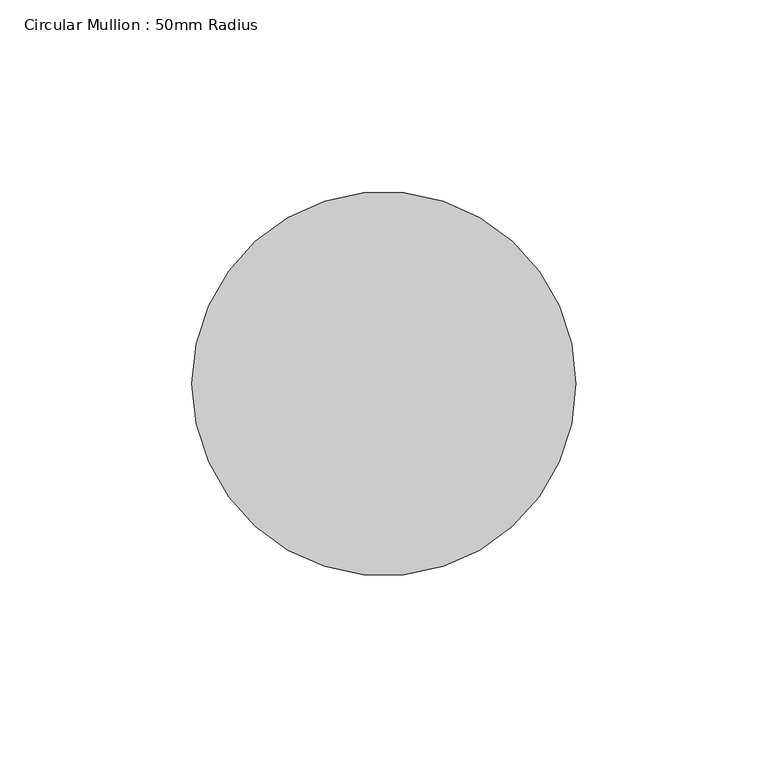
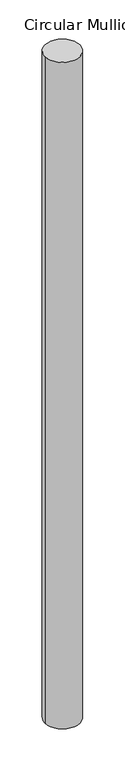
"""IFC4 building model written with IfcOpenShell, lengths in millimetres: member geometry, Circular Mullion : 50mm Radius."""

from ifc_helpers import new_model, si_unit, point, frame, frame_2d, origin, place, context, project, spatial, circle_curve, trimmed, segment, composite_curve, outline, extrude, source, transform, mapped, element, save


def circular_mullion_50mm_radius_da103a8c(model_context):
    return source(origin(), model_context, "Body", "SweptSolid", [
        extrude(outline(composite_curve([segment(trimmed(circle_curve(frame_2d((-50.0, 0.0)), 50.0), [point((0.0, 0.0))], [point((-100.0, 0.0))], False, "CARTESIAN"), True, "CONTINUOUS"), segment(trimmed(circle_curve(frame_2d((-50.0, 0.0)), 50.0), [point((-100.0, 0.0))], [point((0.0, 0.0))], False, "CARTESIAN"), True, "CONTINUOUS")], self_intersect=False)), frame((0.0, 0.0, -2006.0821328), z_axis=(0.0, 0.0, 1.0), x_axis=(1.0, 0.0, 0.0)), (0.0, 0.0, 1.0), 2006.0821328),
    ])


if __name__ == "__main__":
    model = new_model("IFC4")
    model_context = context("Model", 3, world=origin())
    ifc_project = project(units=[si_unit("LENGTHUNIT", "METRE", prefix="MILLI")], contexts=[model_context])
    site = spatial("IfcSite", under=ifc_project)
    building = spatial("IfcBuilding", under=site)
    placement = place(None, origin())
    circular_mullion_50mm_radius_shape = circular_mullion_50mm_radius_da103a8c(model_context)
    element("IfcMember", 1, ObjectType="Circular Mullion : 50mm Radius", at=placement, inside=building, context=model_context, shape_type="MappedRepresentation", body=[
        mapped(circular_mullion_50mm_radius_shape, transform((0.0, 0.0, 0.0), x_axis=(1.0, 0.0, 0.0), y_axis=(0.0, 1.0, 0.0), z_axis=(0.0, 0.0, 1.0))),
    ])
    save(model, "model.ifc")

# Revit data of these elements
# Type "Circular Mullion : 50mm Radius"
#   built-in parameter 1007350 = 0.164042 (stored number, unit not read)
# Element 1 (IfcMember, "Circular Mullion : 50mm Radius")
#   Materials on its faces: "Aluminium"
# Materials
#   "Aluminium": class "Metal", colour RGB 247 247 247, transparency 0, Description = "Aluminium 6061", Cost = 0
